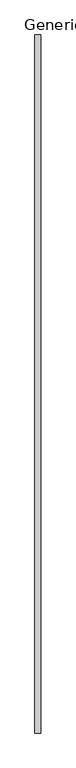
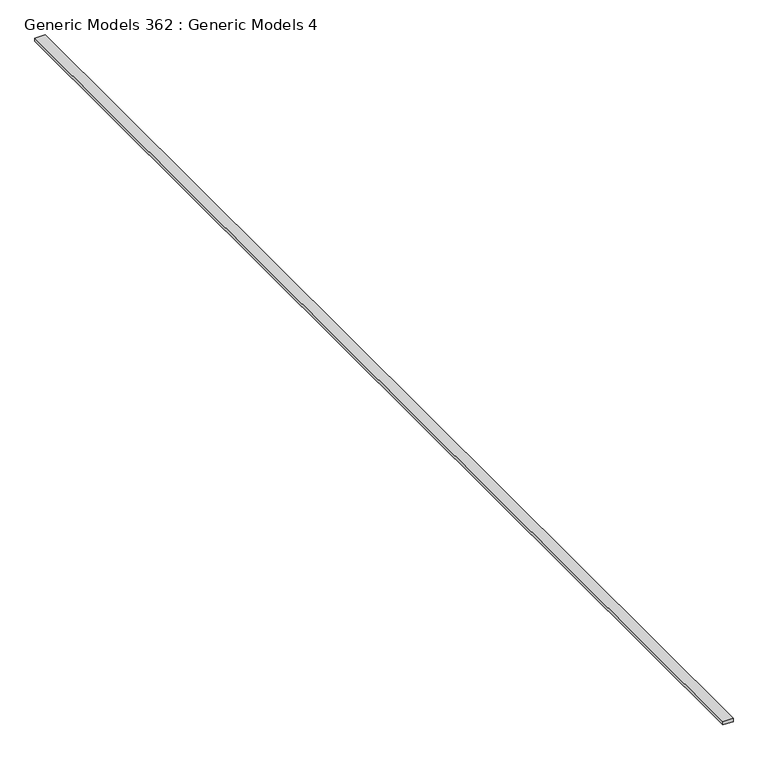
"""IFC4 building model written with IfcOpenShell, lengths in millimetres: proxy geometry, Generic Models 362 : Generic Models 4."""

from ifc_helpers import new_model, si_unit, frame, origin, place, context, project, spatial, polyline, outline, extrude, source, transform, mapped, element, save


def generic_models_362_generic_models_4_487f1ed6(model_context):
    return source(origin(), model_context, "Body", "SweptSolid", [
        extrude(outline(polyline([(-6541.0889404, -6864.9230338), (-6595.6971514, -6864.9230338), (-6595.6971514, -464.1230338), (-6541.0889404, -464.1230338), (-6541.0889404, -6864.9230338)])), frame((0.0, 0.0, 126233.4695142), z_axis=(0.0, 0.0, 1.0), x_axis=(1.0, 0.0, 0.0)), (0.0, 0.0, 1.0), 17.5140645),
    ])


if __name__ == "__main__":
    model = new_model("IFC4")
    model_context = context("Model", 3, world=origin())
    ifc_project = project(units=[si_unit("LENGTHUNIT", "METRE", prefix="MILLI")], contexts=[model_context])
    site = spatial("IfcSite", under=ifc_project)
    building = spatial("IfcBuilding", under=site)
    placement = place(None, origin())
    generic_models_362_generic_models_4_shape = generic_models_362_generic_models_4_487f1ed6(model_context)
    element("IfcBuildingElementProxy", 1, Name="Generic Models 362 : Generic Models 4", ObjectType="Generic Models 362 : Generic Models 4", at=placement, inside=building, context=model_context, shape_type="MappedRepresentation", body=[
        mapped(generic_models_362_generic_models_4_shape, transform((0.0, 0.0, 0.0), x_axis=(1.0, 0.0, 0.0), y_axis=(0.0, 1.0, 0.0), z_axis=(0.0, 0.0, 1.0))),
    ])
    save(model, "model.ifc")

# Revit data of these elements
# Element 1 (IfcBuildingElementProxy, "Generic Models 362 : Generic Models 4")
#   Materials on its faces: "_2X BLOCKING AS REQUIRED"
# Materials
#   "_2X BLOCKING AS REQUIRED": class "Generic", colour RGB 177 130 114, transparency 0, Cost = 0
